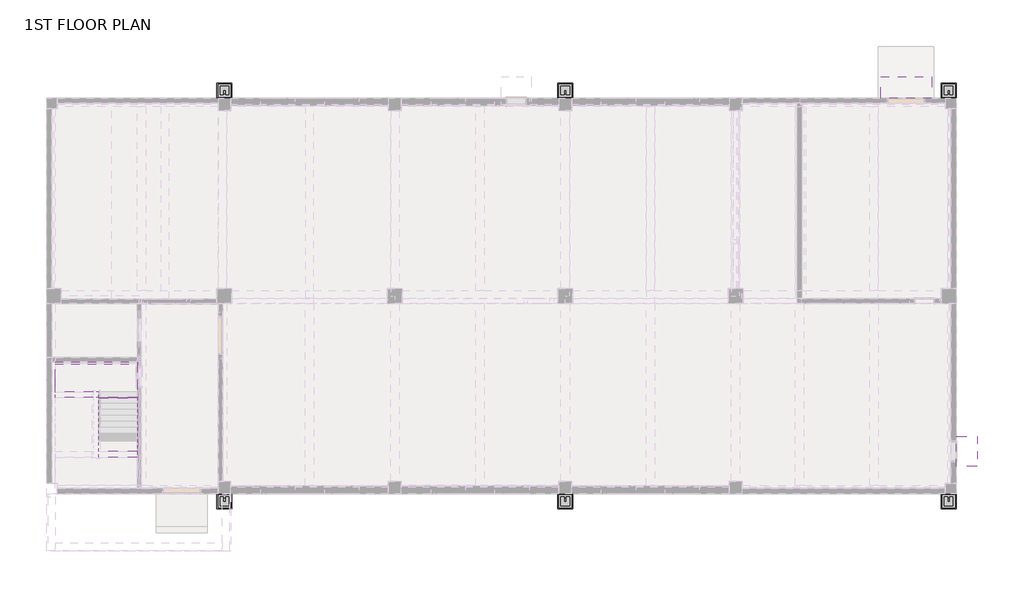
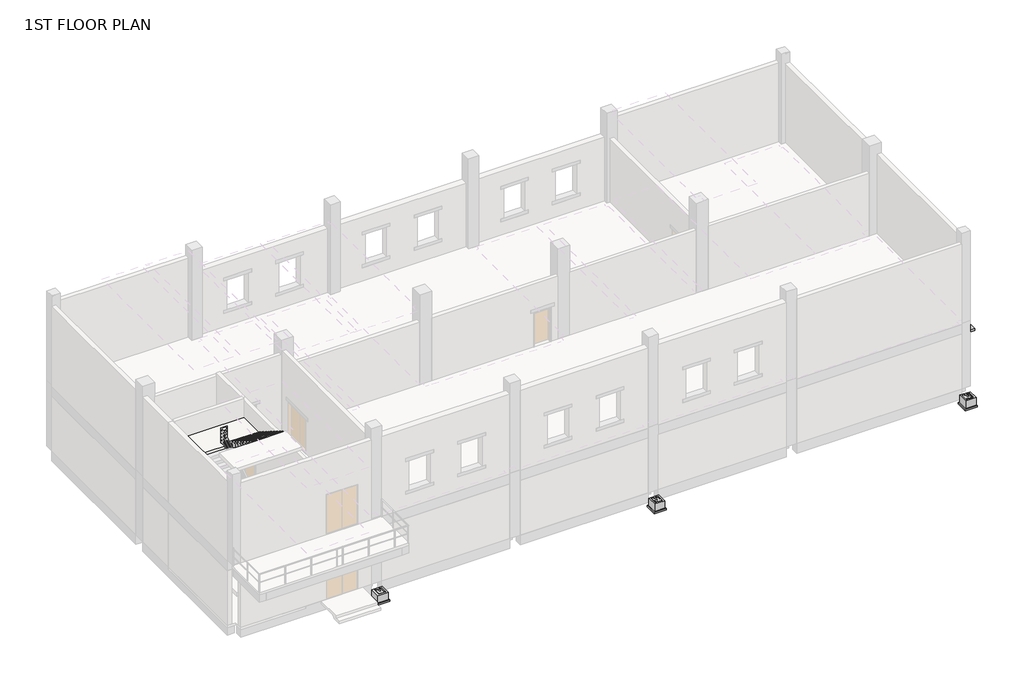
# One storey, part 9 of 9: 8 proxies, 2 slabs, 2 stair flights.
"""IFC4 building model written with IfcOpenShell, lengths in millimetres."""

import ifcopenshell
import ifcopenshell.guid

model = None  # the IFC model being written
_history = None  # IfcOwnerHistory: only IFC2X3 demands one
_inside = {}  # id of a spatial element -> (the spatial element, [elements in it])
_under = {}  # id of a project, library or spatial element -> (it, [spatial elements below it])
_declared = {}  # id of a project -> (the project, [libraries it declares])
_typed = {}  # id of a type object -> (the type object, [elements of that type])
_made_of = {}  # id of a material, layer set ... -> (it, [elements and type objects made of it])


def new_model(schema):
    """Start an empty IFC model of exactly this schema.

    Asked for "IFC4X3", IfcOpenShell would pick the latest addendum, in which some entities
    have other attributes; the version numbers below select the first issue.
    IFC2X3 requires an IfcOwnerHistory on every rooted entity: one is made here for all.
    """
    global model, _history
    if schema == "IFC4X3":
        model = ifcopenshell.file(schema_version=(4, 3, 0, 0))
    else:
        model = ifcopenshell.file(schema=schema)
    _inside.clear()
    _under.clear()
    _declared.clear()
    _typed.clear()
    _made_of.clear()
    _history = None
    if model.schema == "IFC2X3":
        org = make("IfcOrganization", Name="unknown")
        user = make(
            "IfcPersonAndOrganization",
            ThePerson=make("IfcPerson", FamilyName="unknown"),
            TheOrganization=org,
        )
        app = make(
            "IfcApplication",
            ApplicationDeveloper=org,
            Version="unknown",
            ApplicationFullName="unknown",
            ApplicationIdentifier="unknown",
        )
        _history = make(
            "IfcOwnerHistory",
            OwningUser=user,
            OwningApplication=app,
            ChangeAction="ADDED",
            CreationDate=0,
        )
    return model


def make(cls, **values):
    """One entity of the class cls with the attributes given. An attribute that is None is left unset."""
    return model.create_entity(
        cls, **{name: value for name, value in values.items() if value is not None}
    )


def rooted(cls, **values):
    """An entity with a GlobalId (a new one), such as an element, a storey or a relation."""
    return make(cls, GlobalId=ifcopenshell.guid.new(), OwnerHistory=_history, **values)


def si_unit(unit_type, name, prefix=None):
    """IfcSIUnit, for example si_unit("LENGTHUNIT", "METRE", prefix="MILLI")."""
    return make("IfcSIUnit", UnitType=unit_type, Prefix=prefix, Name=name)


def assignment(units):
    """IfcUnitAssignment: the units of a project."""
    return None if units is None else make("IfcUnitAssignment", Units=units)


def point(xyz):
    """IfcCartesianPoint."""
    return None if xyz is None else make("IfcCartesianPoint", Coordinates=xyz)


def direction(xyz):
    """IfcDirection."""
    return None if xyz is None else make("IfcDirection", DirectionRatios=xyz)


def frame(location, z_axis=None, x_axis=None):
    """IfcAxis2Placement3D, a coordinate frame: its origin and axes. An axis left out is left unset."""
    return make(
        "IfcAxis2Placement3D",
        Location=point(location),
        Axis=direction(z_axis),
        RefDirection=direction(x_axis),
    )


def origin():
    """The frame at (0, 0, 0) with its axes left unset."""
    return frame((0.0, 0.0, 0.0))


def origin_with_axes():
    """The frame at (0, 0, 0) with the z axis (0, 0, 1) and the x axis (1, 0, 0) written out."""
    return frame((0.0, 0.0, 0.0), z_axis=(0.0, 0.0, 1.0), x_axis=(1.0, 0.0, 0.0))


def place(relative_to, where):
    """IfcLocalPlacement: puts the frame where relative to a parent placement (None: the world)."""
    return make(
        "IfcLocalPlacement", PlacementRelTo=relative_to, RelativePlacement=where
    )


def context(
    kind, dimensions, precision=None, world=None, true_north=None, identifier=None
):
    """IfcGeometricRepresentationContext, for example the 3D "Model" context."""
    return make(
        "IfcGeometricRepresentationContext",
        ContextIdentifier=identifier,
        ContextType=kind,
        CoordinateSpaceDimension=dimensions,
        Precision=precision,
        WorldCoordinateSystem=world,
        TrueNorth=true_north,
    )


def project(units=None, contexts=None):
    """IfcProject with its units and contexts."""
    return rooted(
        "IfcProject",
        Name="project",
        RepresentationContexts=contexts,
        UnitsInContext=assignment(units),
    )


def spatial(cls, under=None, at=None, **own):
    """A site, building, storey or space (cls), placed at a placement, below another one or the project."""
    s = rooted(cls, ObjectPlacement=at, **own)
    if under is not None:
        _under.setdefault(under.id(), (under, []))[1].append(s)
    return s


def polyline(points):
    """IfcPolyline through the points."""
    return make("IfcPolyline", Points=[point(p) for p in points])


def outline(outer, holes=None, kind="AREA"):
    """IfcArbitraryClosedProfileDef: a profile drawn as a closed curve; with holes, ...WithVoids."""
    if holes is None:
        return make("IfcArbitraryClosedProfileDef", ProfileType=kind, OuterCurve=outer)
    return make(
        "IfcArbitraryProfileDefWithVoids",
        ProfileType=kind,
        OuterCurve=outer,
        InnerCurves=holes,
    )


def extrude(swept, where, along, depth):
    """IfcExtrudedAreaSolid: the profile swept, set in the frame where, extruded along a direction by depth."""
    return make(
        "IfcExtrudedAreaSolid",
        SweptArea=swept,
        Position=where,
        ExtrudedDirection=direction(along),
        Depth=depth,
    )


def faces_of(points, faces, orient=None, outer=None):
    """IfcFace entities. A face is a list of loops; a loop is a list of indices into points, from 0.

    orient and outer hold one flag for each loop. By default every Orientation is true, the
    first loop of a face is its IfcFaceOuterBound and the others are IfcFaceBound.
    """
    made = []
    for i, loops in enumerate(faces):
        bounds = []
        for j, loop in enumerate(loops):
            is_outer = j == 0 if outer is None else outer[i][j]
            bounds.append(
                make(
                    "IfcFaceOuterBound" if is_outer else "IfcFaceBound",
                    Bound=make("IfcPolyLoop", Polygon=[points[k] for k in loop]),
                    Orientation=True if orient is None else orient[i][j],
                )
            )
        made.append(make("IfcFace", Bounds=bounds))
    return made


def faceted_brep(points, faces, orient=None, outer=None, voids=None):
    """IfcFacetedBrep: a solid bounded by flat faces; with voids (closed shells), ...WithVoids."""
    shared = [point(p) for p in points]
    hull = make("IfcClosedShell", CfsFaces=faces_of(shared, faces, orient, outer))
    if voids is None:
        return make("IfcFacetedBrep", Outer=hull)
    return make(
        "IfcFacetedBrepWithVoids",
        Outer=hull,
        Voids=[
            make(cls, CfsFaces=faces_of(shared, fs, o, b)) for cls, fs, o, b in voids
        ],
    )


def shape(context_of_items, identifier, shape_type, items):
    """IfcShapeRepresentation: the items that make up one representation, for example the "Body"."""
    return make(
        "IfcShapeRepresentation",
        ContextOfItems=context_of_items,
        RepresentationIdentifier=identifier,
        RepresentationType=shape_type,
        Items=items,
    )


def source(mapping_origin, context_of_items, identifier, shape_type, items):
    """IfcRepresentationMap: a shape defined once, which mapped items show again and again."""
    return make(
        "IfcRepresentationMap",
        MappingOrigin=mapping_origin,
        MappedRepresentation=shape(context_of_items, identifier, shape_type, items),
    )


def transform(
    local_origin,
    x_axis=None,
    y_axis=None,
    z_axis=None,
    scale=None,
    scale2=None,
    scale3=None,
    uniform=True,
):
    """IfcCartesianTransformationOperator3D, or its non-uniform kind. x_axis, y_axis, z_axis: its Axis1, 2, 3."""
    if uniform:
        return make(
            "IfcCartesianTransformationOperator3D",
            Axis1=direction(x_axis),
            Axis2=direction(y_axis),
            LocalOrigin=point(local_origin),
            Scale=scale,
            Axis3=direction(z_axis),
        )
    return make(
        "IfcCartesianTransformationOperator3DnonUniform",
        Axis1=direction(x_axis),
        Axis2=direction(y_axis),
        LocalOrigin=point(local_origin),
        Scale=scale,
        Axis3=direction(z_axis),
        Scale2=scale2,
        Scale3=scale3,
    )


def mapped(mapping_source, mapping_target):
    """IfcMappedItem: shows the shape of a source again, moved by a transform."""
    return make(
        "IfcMappedItem", MappingSource=mapping_source, MappingTarget=mapping_target
    )


def made_of(thing, what):
    """Note that an element or type object is made of a material, layer set ...; save() writes the relation."""
    if what is not None:
        _made_of.setdefault(what.id(), (what, []))[1].append(thing)
    return thing


def element(
    cls,
    number,
    at=None,
    inside=None,
    cuts=None,
    type_object=None,
    material=None,
    context=None,
    identifier="Body",
    shape_type=None,
    held_by="IfcProductDefinitionShape",
    body=None,
    shapes=None,
    **own,
):
    """One element of the class cls, such as IfcWall. Its Tag is "e" and its number.

    at: its placement. inside: the storey or other place that contains it. cuts: it is an
    opening in that element (IfcRelVoidsElement). A single representation is given by context,
    identifier, shape_type and body (its items); several are given by shapes. held_by: the class
    of the entity that holds the representations. save() writes the other relations.
    """
    e = rooted(cls, Tag="e%d" % number, ObjectPlacement=at, **own)
    if body is not None:
        shapes = [shape(context, identifier, shape_type, body)]
    if shapes is not None:
        e.Representation = make(held_by, Representations=shapes)
    if inside is not None:
        _inside.setdefault(inside.id(), (inside, []))[1].append(e)
    if cuts is not None:
        rooted(
            "IfcRelVoidsElement", RelatingBuildingElement=cuts, RelatedOpeningElement=e
        )
    if type_object is not None:
        _typed.setdefault(type_object.id(), (type_object, []))[1].append(e)
    return made_of(e, material)


def aggregate(whole, parts):
    """IfcRelAggregates: a whole, such as a stair, and the parts it consists of."""
    return rooted("IfcRelAggregates", RelatingObject=whole, RelatedObjects=parts)


def save(model, path):
    """Write the relations noted so far, then the file.

    IfcRelAggregates (storeys below a building ...), IfcRelContainedInSpatialStructure (elements
    in a storey), IfcRelDefinesByType, IfcRelAssociatesMaterial and IfcRelDeclares: one each for
    every whole, place, type object, material and project.
    """
    for whole, parts in _under.values():
        aggregate(whole, parts)
    for where, things in _inside.values():
        rooted(
            "IfcRelContainedInSpatialStructure",
            RelatedElements=things,
            RelatingStructure=where,
        )
    for kind, things in _typed.values():
        rooted("IfcRelDefinesByType", RelatedObjects=things, RelatingType=kind)
    for what, things in _made_of.values():
        rooted("IfcRelAssociatesMaterial", RelatedObjects=things, RelatingMaterial=what)
    for by, libraries in _declared.values():
        rooted("IfcRelDeclares", RelatingContext=by, RelatedDefinitions=libraries)
    model.write(path)


def generic_models_4b8b6a59(model_context):
    return source(origin(), model_context, "Body", "SolidModel", [
        extrude(outline(polyline([(-55.0, 140.0), (-55.0, 132.0), (-132.0, 132.0), (-132.0, -132.0), (132.0, -132.0), (132.0, 132.0), (55.0, 132.0), (55.0, 140.0), (140.0, 140.0), (140.0, -140.0), (-140.0, -140.0), (-140.0, 140.0), (-55.0, 140.0)])), frame((0.0, 0.0, -10.0), z_axis=(0.0, 0.0, 1.0), x_axis=(1.0, 0.0, 0.0)), (0.0, 0.0, 1.0), 10.0),
        extrude(outline(polyline([(-55.0, 200.0), (-55.0, -20.0), (55.0, -20.0), (55.0, 200.0), (200.0, 200.0), (200.0, -200.0), (-200.0, -200.0), (-200.0, 200.0), (-55.0, 200.0)])), origin_with_axes(), (0.0, 0.0, 1.0), 8.0),
        faceted_brep([(150.0, -150.0, -300.0), (150.0, 150.0, -300.0), (-150.0, 150.0, -300.0), (-150.0, -150.0, -300.0), (300.0, 300.0, -450.0), (300.0, -300.0, -450.0), (-300.0, -300.0, -450.0), (-300.0, 300.0, -450.0), (-300.0, 300.0, 0.0), (300.0, 300.0, 0.0), (-300.0, -300.0, 0.0), (300.0, -300.0, 0.0), (150.0, 150.0, 0.0), (150.0, -150.0, 0.0), (-150.0, -150.0, 0.0), (-150.0, 150.0, 0.0)], [[[0, 1, 2, 3]], [[4, 5, 6, 7]], [[4, 7, 8, 9]], [[8, 7, 6, 10]], [[10, 6, 5, 11]], [[11, 5, 4, 9]], [[9, 8, 10, 11], [12, 13, 14, 15]], [[13, 12, 1, 0]], [[14, 13, 0, 3]], [[15, 14, 3, 2]], [[12, 15, 2, 1]]]),
        extrude(outline(polyline([(350.0, 350.0), (350.0, -350.0), (-350.0, -350.0), (-350.0, 350.0), (350.0, 350.0)])), frame((0.0, 0.0, -550.0), z_axis=(0.0, 0.0, 1.0), x_axis=(1.0, 0.0, 0.0)), (0.0, 0.0, 1.0), 100.0),
    ])


def generic_models_1eaa761a(model_context):
    return source(origin(), model_context, "Body", "SolidModel", [
        extrude(outline(polyline([(-55.0, -140.0), (-140.0, -140.0), (-140.0, 140.0), (140.0, 140.0), (140.0, -140.0), (55.0, -140.0), (55.0, -132.0), (132.0, -132.0), (132.0, 132.0), (-132.0, 132.0), (-132.0, -132.0), (-55.0, -132.0), (-55.0, -140.0)])), frame((0.0, 0.0, -10.0), z_axis=(0.0, 0.0, 1.0), x_axis=(1.0, 0.0, 0.0)), (0.0, 0.0, 1.0), 10.0),
        extrude(outline(polyline([(-55.0, -200.0), (-200.0, -200.0), (-200.0, 200.0), (200.0, 200.0), (200.0, -200.0), (55.0, -200.0), (55.0, 20.0), (-55.0, 20.0), (-55.0, -200.0)])), origin_with_axes(), (0.0, 0.0, 1.0), 8.0),
        faceted_brep([(150.0, 150.0, -300.0), (-150.0, 150.0, -300.0), (-150.0, -150.0, -300.0), (150.0, -150.0, -300.0), (300.0, -300.0, -450.0), (-300.0, -300.0, -450.0), (-300.0, 300.0, -450.0), (300.0, 300.0, -450.0), (300.0, -300.0, 0.0), (-300.0, -300.0, 0.0), (-300.0, 300.0, 0.0), (300.0, 300.0, 0.0), (150.0, -150.0, 0.0), (-150.0, -150.0, 0.0), (-150.0, 150.0, 0.0), (150.0, 150.0, 0.0)], [[[0, 1, 2, 3]], [[4, 5, 6, 7]], [[4, 8, 9, 5]], [[9, 10, 6, 5]], [[10, 11, 7, 6]], [[11, 8, 4, 7]], [[8, 11, 10, 9], [12, 13, 14, 15]], [[15, 0, 3, 12]], [[14, 1, 0, 15]], [[13, 2, 1, 14]], [[12, 3, 2, 13]]]),
        extrude(outline(polyline([(350.0, -350.0), (-350.0, -350.0), (-350.0, 350.0), (350.0, 350.0), (350.0, -350.0)])), frame((0.0, 0.0, -550.0), z_axis=(0.0, 0.0, 1.0), x_axis=(1.0, 0.0, 0.0)), (0.0, 0.0, 1.0), 100.0),
    ])


def canopy_no_lintel2_canopy_no_lintel_90d8ac49(model_context):
    return source(origin(), model_context, "Body", "SweptSolid", [
        extrude(outline(polyline([(-30.0, 1000.0), (0.0, 0.0), (-150.0, 0.0), (-150.0, 1000.0), (-30.0, 1000.0)])), frame((0.0, 0.0, 0.0), z_axis=(1.0, 0.0, 0.0), x_axis=(0.0, 1.0, 0.0)), (0.0, 0.0, 1.0), 1400.0),
    ])


def canopy_no_lintel2_canopy_no_lintel_c6626c79(model_context):
    return source(origin(), model_context, "Body", "SweptSolid", [
        extrude(outline(polyline([(-30.0, 1000.0), (0.0, 0.0), (-150.0, 0.0), (-150.0, 1000.0), (-30.0, 1000.0)])), frame((0.0, 0.0, 0.0), z_axis=(1.0, 0.0, 0.0), x_axis=(0.0, 1.0, 0.0)), (0.0, 0.0, 1.0), 2400.0),
    ])


model = new_model("IFC4")

# Units and contexts
model_context = context("Model", 3, world=origin())
ifc_project = project(units=[si_unit("LENGTHUNIT", "METRE", prefix="MILLI")], contexts=[model_context])

# Site, building, storey
site = spatial("IfcSite", under=ifc_project)
building = spatial("IfcBuilding", under=site)
storey = spatial("IfcBuildingStorey", under=building, Name="1ST FLOOR PLAN", Elevation=600.005241)

# Proxies
placement = place(None, origin())
generic_models_shape = generic_models_4b8b6a59(model_context)
element("IfcBuildingElementProxy", 1, Name="Catchpit : Rainwater Catchpit", ObjectType="Catchpit : Rainwater Catchpit", at=placement, inside=storey, context=model_context, shape_type="MappedRepresentation", body=[
    mapped(generic_models_shape, transform((8000.0, 20349.4942467, 300.005241), x_axis=(1.0, 0.0, 0.0), y_axis=(0.0, 1.0, 0.0), z_axis=(0.0, 0.0, 1.0))),
])
element("IfcBuildingElementProxy", 2, Name="Catchpit : Rainwater Catchpit", ObjectType="Catchpit : Rainwater Catchpit", at=placement, inside=storey, context=model_context, shape_type="MappedRepresentation", body=[
    mapped(generic_models_shape, transform((24000.0, 20349.4942467, 300.005241), x_axis=(1.0, 0.0, 0.0), y_axis=(0.0, 1.0, 0.0), z_axis=(0.0, 0.0, 1.0))),
])
element("IfcBuildingElementProxy", 3, Name="Catchpit : Rainwater Catchpit", ObjectType="Catchpit : Rainwater Catchpit", at=placement, inside=storey, context=model_context, shape_type="MappedRepresentation", body=[
    mapped(generic_models_shape, transform((42000.0, 20349.4942467, 300.005241), x_axis=(1.0, 0.0, 0.0), y_axis=(0.0, 1.0, 0.0), z_axis=(0.0, 0.0, 1.0))),
])
generic_models_2_shape = generic_models_1eaa761a(model_context)
element("IfcBuildingElementProxy", 4, Name="Catchpit : Rainwater Catchpit", ObjectType="Catchpit : Rainwater Catchpit", at=placement, inside=storey, context=model_context, shape_type="MappedRepresentation", body=[
    mapped(generic_models_2_shape, transform((8000.0, 39649.5474711, 300.005241), x_axis=(1.0, 0.0, 0.0), y_axis=(0.0, 1.0, 0.0), z_axis=(0.0, 0.0, 1.0))),
])
element("IfcBuildingElementProxy", 5, Name="Catchpit : Rainwater Catchpit", ObjectType="Catchpit : Rainwater Catchpit", at=placement, inside=storey, context=model_context, shape_type="MappedRepresentation", body=[
    mapped(generic_models_2_shape, transform((24000.0, 39649.5474711, 300.005241), x_axis=(1.0, 0.0, 0.0), y_axis=(0.0, 1.0, 0.0), z_axis=(0.0, 0.0, 1.0))),
])
element("IfcBuildingElementProxy", 6, Name="Catchpit : Rainwater Catchpit", ObjectType="Catchpit : Rainwater Catchpit", at=placement, inside=storey, context=model_context, shape_type="MappedRepresentation", body=[
    mapped(generic_models_2_shape, transform((42000.0, 39649.5474711, 300.005241), x_axis=(1.0, 0.0, 0.0), y_axis=(0.0, 1.0, 0.0), z_axis=(0.0, 0.0, 1.0))),
])
canopy_no_lintel2_canopy_no_lintel_shape = canopy_no_lintel2_canopy_no_lintel_90d8ac49(model_context)
element("IfcBuildingElementProxy", 7, Name="Canopy_no_ Lintel2 : Canopy No Lintel", ObjectType="Canopy_no_ Lintel2 : Canopy No Lintel", at=placement, inside=storey, context=model_context, shape_type="MappedRepresentation", body=[
    mapped(canopy_no_lintel2_canopy_no_lintel_shape, transform((42351.0, 21999.5208589, 3000.005241), x_axis=(0.0, 1.0, 0.0), y_axis=(0.0, 0.0, 1.0), z_axis=(1.0, 0.0, 0.0))),
])
canopy_no_lintel2_canopy_no_lintel_2_shape = canopy_no_lintel2_canopy_no_lintel_c6626c79(model_context)
element("IfcBuildingElementProxy", 8, Name="Canopy_no_ Lintel2 : Canopy No Lintel", ObjectType="Canopy_no_ Lintel2 : Canopy No Lintel", at=placement, inside=storey, context=model_context, shape_type="MappedRepresentation", body=[
    mapped(canopy_no_lintel2_canopy_no_lintel_2_shape, transform((41200.0, 39300.5208589, 3400.005241), x_axis=(-1.0, 0.0, 0.0), y_axis=(0.0, 0.0, 1.0), z_axis=(0.0, 1.0, 0.0))),
])

# Slabs
element("IfcSlab", 9, ObjectType="프리캐스트 콘크리트 - 200mm 두께", at=placement, inside=storey, context=model_context, shape_type="SolidModel", body=[
    faceted_brep([(50.0, 25499.5208589, 4599.211491), (1850.0, 25499.5208589, 4599.211491), (2100.0, 25499.5208589, 4599.211491), (2100.0, 25219.5208589, 4599.211491), (3900.0, 25219.5208589, 4599.211491), (3900.0, 26799.5208589, 4599.211491), (50.0, 26799.5208589, 4599.211491), (50.0, 25736.7852447, 4599.211491), (3900.0, 25219.5208589, 4399.211491), (3900.0, 26799.5208589, 4399.211491), (50.0, 26799.5208589, 4399.211491), (50.0, 25499.5208589, 4257.9826899), (50.0, 25499.5208589, 4432.5448243), (50.0, 25736.7852447, 4399.211491), (1850.0, 25736.7852447, 4399.211491), (2100.0, 25219.5208589, 4399.211491), (2100.0, 25499.5208589, 4399.211491), (1850.0, 25499.5208589, 4399.211491), (1850.0, 25499.5208589, 4257.9826899)], [[[0, 1, 2, 3, 4, 5, 6, 7]], [[5, 4, 8, 9]], [[6, 5, 9, 10]], [[11, 12, 0, 7, 6, 10, 13]], [[14, 13, 10, 9, 8, 15, 16, 17]], [[1, 0, 12, 11, 18, 17]], [[2, 1, 17, 16]], [[13, 14, 18, 11]], [[14, 17, 18]], [[3, 2, 16, 15]], [[4, 3, 15, 8]]]),
    extrude(outline(polyline([(50.0, 25499.5208589), (50.0, 26799.5208589), (3900.0, 26799.5208589), (3900.0, 25219.5208589), (2100.0, 25219.5208589), (2100.0, 25499.5208589), (1850.0, 25499.5208589), (50.0, 25499.5208589)])), frame((0.0, 0.0, 4599.211491), z_axis=(0.0, 0.0, 1.0), x_axis=(1.0, 0.0, 0.0)), (0.0, 0.0, 1.0), 0.79375),
])
element("IfcSlab", 10, ObjectType="프리캐스트 콘크리트 - 200mm 두께", at=placement, inside=storey, context=model_context, shape_type="SolidModel", body=[
    faceted_brep([(50.0, 25219.5208589, 8380.461491), (1850.0, 25219.5208589, 8380.461491), (2100.0, 25219.5208589, 8380.461491), (3900.0, 25219.5208589, 8380.461491), (3900.0, 25258.6099233, 8380.461491), (3900.0, 26899.5208589, 8380.461491), (50.0, 26899.5208589, 8380.461491), (50.0, 25460.4317945, 8380.461491), (50.0, 25219.5208589, 8208.586491), (50.0, 25219.5208589, 8032.5808943), (1850.0, 25219.5208589, 8032.5808943), (1850.0, 25219.5208589, 8180.461491), (2100.0, 25219.5208589, 8180.461491), (2100.0, 25219.5208589, 8204.4558943), (3900.0, 25219.5208589, 8204.4558943), (3900.0, 25258.6099233, 8180.461491), (3900.0, 26899.5208589, 8180.461491), (50.0, 26899.5208589, 8180.461491), (50.0, 25460.4317945, 8180.461491), (2100.0, 25258.6099233, 8180.461491), (1850.0, 25460.4317945, 8180.461491)], [[[0, 1, 2, 3, 4, 5, 6, 7]], [[1, 0, 8, 9, 10, 11]], [[2, 1, 11, 12, 13]], [[3, 2, 13, 14]], [[3, 14, 15, 16, 5, 4]], [[6, 5, 16, 17]], [[9, 8, 0, 7, 6, 17, 18]], [[19, 12, 11, 20, 18, 17, 16, 15]], [[12, 19, 13]], [[18, 20, 10, 9]], [[20, 11, 10]], [[19, 15, 14, 13]]]),
    extrude(outline(polyline([(50.0, 25219.5208589), (50.0, 26899.5208589), (3900.0, 26899.5208589), (3900.0, 25219.5208589), (2100.0, 25219.5208589), (1850.0, 25219.5208589), (50.0, 25219.5208589)])), frame((0.0, 0.0, 8380.461491), z_axis=(0.0, 0.0, 1.0), x_axis=(1.0, 0.0, 0.0)), (0.0, 0.0, 1.0), 0.79375),
])

# Stair flights
element("IfcStairFlight", 11, ObjectType="1mm 디딤판", at=placement, inside=storey, context=model_context, shape_type="SolidModel", body=[
    faceted_brep([(3900.0, 24939.5208589, 4771.086491), (3900.0, 25219.5208589, 4771.086491), (2100.0, 25219.5208589, 4771.086491), (2100.0, 24939.5208589, 4771.086491), (3900.0, 24939.5208589, 4600.005241), (3900.0, 25219.5208589, 4600.005241), (2100.0, 25219.5208589, 4600.005241), (2100.0, 24939.5208589, 4600.005241), (3900.0, 24659.5208589, 4942.961491), (3900.0, 24939.5208589, 4942.961491), (2100.0, 24939.5208589, 4942.961491), (2100.0, 24659.5208589, 4942.961491), (3900.0, 24659.5208589, 4766.9558943), (3900.0, 24931.4986506, 4600.005241), (2100.0, 24931.4986506, 4600.005241), (2100.0, 24659.5208589, 4766.9558943), (3900.0, 24379.5208589, 5114.836491), (3900.0, 24659.5208589, 5114.836491), (2100.0, 24659.5208589, 5114.836491), (2100.0, 24379.5208589, 5114.836491), (3900.0, 24379.5208589, 4938.8308943), (2100.0, 24379.5208589, 4938.8308943), (3900.0, 24099.5208589, 5286.711491), (3900.0, 24379.5208589, 5286.711491), (2100.0, 24379.5208589, 5286.711491), (2100.0, 24099.5208589, 5286.711491), (3900.0, 24099.5208589, 5110.7058943), (2100.0, 24099.5208589, 5110.7058943), (3900.0, 23819.5208589, 5458.586491), (3900.0, 24099.5208589, 5458.586491), (2100.0, 24099.5208589, 5458.586491), (2100.0, 23819.5208589, 5458.586491), (3900.0, 23819.5208589, 5282.5808943), (2100.0, 23819.5208589, 5282.5808943), (3900.0, 23539.5208589, 5630.461491), (3900.0, 23819.5208589, 5630.461491), (2100.0, 23819.5208589, 5630.461491), (2100.0, 23539.5208589, 5630.461491), (3900.0, 23539.5208589, 5454.4558943), (2100.0, 23539.5208589, 5454.4558943), (3900.0, 23259.5208589, 5802.336491), (3900.0, 23539.5208589, 5802.336491), (2100.0, 23539.5208589, 5802.336491), (2100.0, 23259.5208589, 5802.336491), (3900.0, 23259.5208589, 5626.3308943), (2100.0, 23259.5208589, 5626.3308943), (3900.0, 22979.5208589, 5974.211491), (3900.0, 23259.5208589, 5974.211491), (2100.0, 23259.5208589, 5974.211491), (2100.0, 22979.5208589, 5974.211491), (3900.0, 22979.5208589, 5798.2058943), (2100.0, 22979.5208589, 5798.2058943), (3900.0, 22699.5208589, 6146.086491), (3900.0, 22979.5208589, 6146.086491), (2100.0, 22979.5208589, 6146.086491), (2100.0, 22699.5208589, 6146.086491), (3900.0, 22699.5208589, 5970.0808943), (2100.0, 22699.5208589, 5970.0808943), (3900.0, 22419.5208589, 6317.961491), (3900.0, 22699.5208589, 6317.961491), (2100.0, 22699.5208589, 6317.961491), (2100.0, 22419.5208589, 6317.961491), (3900.0, 22419.5208589, 6141.9558943), (2100.0, 22419.5208589, 6141.9558943), (2100.0, 22419.5208589, 6289.836491)], [[[0, 1, 2, 3]], [[1, 0, 4, 5]], [[2, 1, 5, 6]], [[3, 2, 6, 7]], [[8, 9, 10, 11]], [[4, 0, 9, 8, 12, 13]], [[0, 3, 10, 9]], [[3, 7, 14, 15, 11, 10]], [[16, 17, 18, 19]], [[17, 16, 20, 12, 8]], [[8, 11, 18, 17]], [[19, 18, 11, 15, 21]], [[22, 23, 24, 25]], [[23, 22, 26, 20, 16]], [[16, 19, 24, 23]], [[25, 24, 19, 21, 27]], [[28, 29, 30, 31]], [[29, 28, 32, 26, 22]], [[22, 25, 30, 29]], [[31, 30, 25, 27, 33]], [[34, 35, 36, 37]], [[35, 34, 38, 32, 28]], [[28, 31, 36, 35]], [[37, 36, 31, 33, 39]], [[40, 41, 42, 43]], [[41, 40, 44, 38, 34]], [[34, 37, 42, 41]], [[43, 42, 37, 39, 45]], [[46, 47, 48, 49]], [[47, 46, 50, 44, 40]], [[40, 43, 48, 47]], [[49, 48, 43, 45, 51]], [[52, 53, 54, 55]], [[53, 52, 56, 50, 46]], [[46, 49, 54, 53]], [[55, 54, 49, 51, 57]], [[58, 59, 60, 61]], [[59, 58, 62, 56, 52]], [[52, 55, 60, 59]], [[61, 60, 55, 57, 63, 64]], [[58, 61, 64, 63, 62]], [[5, 4, 13, 14, 7, 6]], [[14, 13, 12, 20, 26, 32, 38, 44, 50, 56, 62, 63, 57, 51, 45, 39, 33, 27, 21, 15]]]),
    extrude(outline(polyline([(3900.0, 24939.5208589), (2100.0, 24939.5208589), (2100.0, 25219.5208589), (3900.0, 25219.5208589), (3900.0, 24939.5208589)])), frame((0.0, 0.0, 4771.086491), z_axis=(0.0, 0.0, 1.0), x_axis=(1.0, 0.0, 0.0)), (0.0, 0.0, 1.0), 0.79375),
    extrude(outline(polyline([(3900.0, 24659.5208589), (2100.0, 24659.5208589), (2100.0, 24939.5208589), (3900.0, 24939.5208589), (3900.0, 24659.5208589)])), frame((0.0, 0.0, 4942.961491), z_axis=(0.0, 0.0, 1.0), x_axis=(1.0, 0.0, 0.0)), (0.0, 0.0, 1.0), 0.79375),
    extrude(outline(polyline([(3900.0, 24379.5208589), (2100.0, 24379.5208589), (2100.0, 24659.5208589), (3900.0, 24659.5208589), (3900.0, 24379.5208589)])), frame((0.0, 0.0, 5114.836491), z_axis=(0.0, 0.0, 1.0), x_axis=(1.0, 0.0, 0.0)), (0.0, 0.0, 1.0), 0.79375),
    extrude(outline(polyline([(3900.0, 24099.5208589), (2100.0, 24099.5208589), (2100.0, 24379.5208589), (3900.0, 24379.5208589), (3900.0, 24099.5208589)])), frame((0.0, 0.0, 5286.711491), z_axis=(0.0, 0.0, 1.0), x_axis=(1.0, 0.0, 0.0)), (0.0, 0.0, 1.0), 0.79375),
    extrude(outline(polyline([(3900.0, 23819.5208589), (2100.0, 23819.5208589), (2100.0, 24099.5208589), (3900.0, 24099.5208589), (3900.0, 23819.5208589)])), frame((0.0, 0.0, 5458.586491), z_axis=(0.0, 0.0, 1.0), x_axis=(1.0, 0.0, 0.0)), (0.0, 0.0, 1.0), 0.79375),
    extrude(outline(polyline([(3900.0, 23539.5208589), (2100.0, 23539.5208589), (2100.0, 23819.5208589), (3900.0, 23819.5208589), (3900.0, 23539.5208589)])), frame((0.0, 0.0, 5630.461491), z_axis=(0.0, 0.0, 1.0), x_axis=(1.0, 0.0, 0.0)), (0.0, 0.0, 1.0), 0.79375),
    extrude(outline(polyline([(3900.0, 23259.5208589), (2100.0, 23259.5208589), (2100.0, 23539.5208589), (3900.0, 23539.5208589), (3900.0, 23259.5208589)])), frame((0.0, 0.0, 5802.336491), z_axis=(0.0, 0.0, 1.0), x_axis=(1.0, 0.0, 0.0)), (0.0, 0.0, 1.0), 0.79375),
    extrude(outline(polyline([(3900.0, 22979.5208589), (2100.0, 22979.5208589), (2100.0, 23259.5208589), (3900.0, 23259.5208589), (3900.0, 22979.5208589)])), frame((0.0, 0.0, 5974.211491), z_axis=(0.0, 0.0, 1.0), x_axis=(1.0, 0.0, 0.0)), (0.0, 0.0, 1.0), 0.79375),
    extrude(outline(polyline([(3900.0, 22699.5208589), (2100.0, 22699.5208589), (2100.0, 22979.5208589), (3900.0, 22979.5208589), (3900.0, 22699.5208589)])), frame((0.0, 0.0, 6146.086491), z_axis=(0.0, 0.0, 1.0), x_axis=(1.0, 0.0, 0.0)), (0.0, 0.0, 1.0), 0.79375),
    extrude(outline(polyline([(3900.0, 22419.5208589), (2100.0, 22419.5208589), (2100.0, 22699.5208589), (3900.0, 22699.5208589), (3900.0, 22419.5208589)])), frame((0.0, 0.0, 6317.961491), z_axis=(0.0, 0.0, 1.0), x_axis=(1.0, 0.0, 0.0)), (0.0, 0.0, 1.0), 0.79375),
])
element("IfcStairFlight", 12, ObjectType="1mm 디딤판", at=placement, inside=storey, context=model_context, shape_type="SolidModel", body=[
    faceted_brep([(3900.0, 24939.5208589, 8552.336491), (3900.0, 25219.5208589, 8552.336491), (2100.0, 25219.5208589, 8552.336491), (2100.0, 24939.5208589, 8552.336491), (3900.0, 24939.5208589, 8376.3308943), (3900.0, 25219.5208589, 8204.4558943), (3900.0, 25219.5208589, 8380.461491), (2100.0, 25219.5208589, 8204.4558943), (2100.0, 24939.5208589, 8376.3308943), (3900.0, 24659.5208589, 8724.211491), (3900.0, 24939.5208589, 8724.211491), (2100.0, 24939.5208589, 8724.211491), (2100.0, 24659.5208589, 8724.211491), (3900.0, 24659.5208589, 8548.2058943), (2100.0, 24659.5208589, 8548.2058943), (3900.0, 24379.5208589, 8896.086491), (3900.0, 24659.5208589, 8896.086491), (2100.0, 24659.5208589, 8896.086491), (2100.0, 24379.5208589, 8896.086491), (3900.0, 24379.5208589, 8720.0808943), (2100.0, 24379.5208589, 8720.0808943), (3900.0, 24099.5208589, 9067.961491), (3900.0, 24379.5208589, 9067.961491), (2100.0, 24379.5208589, 9067.961491), (2100.0, 24099.5208589, 9067.961491), (3900.0, 24099.5208589, 8891.9558943), (2100.0, 24099.5208589, 8891.9558943), (3900.0, 23819.5208589, 9239.836491), (3900.0, 24099.5208589, 9239.836491), (2100.0, 24099.5208589, 9239.836491), (2100.0, 23819.5208589, 9239.836491), (3900.0, 23819.5208589, 9063.8308943), (2100.0, 23819.5208589, 9063.8308943), (3900.0, 23539.5208589, 9411.711491), (3900.0, 23819.5208589, 9411.711491), (2100.0, 23819.5208589, 9411.711491), (2100.0, 23539.5208589, 9411.711491), (3900.0, 23539.5208589, 9235.7058943), (2100.0, 23539.5208589, 9235.7058943), (3900.0, 23259.5208589, 9583.586491), (3900.0, 23539.5208589, 9583.586491), (2100.0, 23539.5208589, 9583.586491), (2100.0, 23259.5208589, 9583.586491), (3900.0, 23259.5208589, 9407.5808943), (2100.0, 23259.5208589, 9407.5808943), (3900.0, 22979.5208589, 9755.461491), (3900.0, 23259.5208589, 9755.461491), (2100.0, 23259.5208589, 9755.461491), (2100.0, 22979.5208589, 9755.461491), (3900.0, 22979.5208589, 9579.4558943), (2100.0, 22979.5208589, 9579.4558943), (3900.0, 22699.5208589, 9927.336491), (3900.0, 22979.5208589, 9927.336491), (2100.0, 22979.5208589, 9927.336491), (2100.0, 22699.5208589, 9927.336491), (3900.0, 22699.5208589, 9751.3308943), (2100.0, 22699.5208589, 9751.3308943), (2100.0, 22699.5208589, 9899.211491)], [[[0, 1, 2, 3]], [[1, 0, 4, 5, 6]], [[2, 1, 6, 5, 7]], [[3, 2, 7, 8]], [[9, 10, 11, 12]], [[10, 9, 13, 4, 0]], [[11, 10, 0, 3]], [[12, 11, 3, 8, 14]], [[15, 16, 17, 18]], [[16, 15, 19, 13, 9]], [[17, 16, 9, 12]], [[18, 17, 12, 14, 20]], [[21, 22, 23, 24]], [[22, 21, 25, 19, 15]], [[23, 22, 15, 18]], [[24, 23, 18, 20, 26]], [[27, 28, 29, 30]], [[28, 27, 31, 25, 21]], [[29, 28, 21, 24]], [[30, 29, 24, 26, 32]], [[33, 34, 35, 36]], [[34, 33, 37, 31, 27]], [[35, 34, 27, 30]], [[36, 35, 30, 32, 38]], [[39, 40, 41, 42]], [[40, 39, 43, 37, 33]], [[41, 40, 33, 36]], [[42, 41, 36, 38, 44]], [[45, 46, 47, 48]], [[46, 45, 49, 43, 39]], [[47, 46, 39, 42]], [[48, 47, 42, 44, 50]], [[51, 52, 53, 54]], [[52, 51, 55, 49, 45]], [[53, 52, 45, 48]], [[54, 53, 48, 50, 56, 57]], [[51, 54, 57, 56, 55]], [[5, 4, 13, 19, 25, 31, 37, 43, 49, 55, 56, 50, 44, 38, 32, 26, 20, 14, 8, 7]]]),
    extrude(outline(polyline([(3900.0, 24939.5208589), (2100.0, 24939.5208589), (2100.0, 25219.5208589), (3900.0, 25219.5208589), (3900.0, 24939.5208589)])), frame((0.0, 0.0, 8552.336491), z_axis=(0.0, 0.0, 1.0), x_axis=(1.0, 0.0, 0.0)), (0.0, 0.0, 1.0), 0.79375),
    extrude(outline(polyline([(3900.0, 24659.5208589), (2100.0, 24659.5208589), (2100.0, 24939.5208589), (3900.0, 24939.5208589), (3900.0, 24659.5208589)])), frame((0.0, 0.0, 8724.211491), z_axis=(0.0, 0.0, 1.0), x_axis=(1.0, 0.0, 0.0)), (0.0, 0.0, 1.0), 0.79375),
    extrude(outline(polyline([(3900.0, 24379.5208589), (2100.0, 24379.5208589), (2100.0, 24659.5208589), (3900.0, 24659.5208589), (3900.0, 24379.5208589)])), frame((0.0, 0.0, 8896.086491), z_axis=(0.0, 0.0, 1.0), x_axis=(1.0, 0.0, 0.0)), (0.0, 0.0, 1.0), 0.79375),
    extrude(outline(polyline([(3900.0, 24099.5208589), (2100.0, 24099.5208589), (2100.0, 24379.5208589), (3900.0, 24379.5208589), (3900.0, 24099.5208589)])), frame((0.0, 0.0, 9067.961491), z_axis=(0.0, 0.0, 1.0), x_axis=(1.0, 0.0, 0.0)), (0.0, 0.0, 1.0), 0.79375),
    extrude(outline(polyline([(3900.0, 23819.5208589), (2100.0, 23819.5208589), (2100.0, 24099.5208589), (3900.0, 24099.5208589), (3900.0, 23819.5208589)])), frame((0.0, 0.0, 9239.836491), z_axis=(0.0, 0.0, 1.0), x_axis=(1.0, 0.0, 0.0)), (0.0, 0.0, 1.0), 0.79375),
    extrude(outline(polyline([(3900.0, 23539.5208589), (2100.0, 23539.5208589), (2100.0, 23819.5208589), (3900.0, 23819.5208589), (3900.0, 23539.5208589)])), frame((0.0, 0.0, 9411.711491), z_axis=(0.0, 0.0, 1.0), x_axis=(1.0, 0.0, 0.0)), (0.0, 0.0, 1.0), 0.79375),
    extrude(outline(polyline([(3900.0, 23259.5208589), (2100.0, 23259.5208589), (2100.0, 23539.5208589), (3900.0, 23539.5208589), (3900.0, 23259.5208589)])), frame((0.0, 0.0, 9583.586491), z_axis=(0.0, 0.0, 1.0), x_axis=(1.0, 0.0, 0.0)), (0.0, 0.0, 1.0), 0.79375),
    extrude(outline(polyline([(3900.0, 22979.5208589), (2100.0, 22979.5208589), (2100.0, 23259.5208589), (3900.0, 23259.5208589), (3900.0, 22979.5208589)])), frame((0.0, 0.0, 9755.461491), z_axis=(0.0, 0.0, 1.0), x_axis=(1.0, 0.0, 0.0)), (0.0, 0.0, 1.0), 0.79375),
    extrude(outline(polyline([(3900.0, 22699.5208589), (2100.0, 22699.5208589), (2100.0, 22979.5208589), (3900.0, 22979.5208589), (3900.0, 22699.5208589)])), frame((0.0, 0.0, 9927.336491), z_axis=(0.0, 0.0, 1.0), x_axis=(1.0, 0.0, 0.0)), (0.0, 0.0, 1.0), 0.79375),
])

save(model, "model.ifc")

# Revit data of these elements
# Type "Catchpit : Rainwater Catchpit"
#   Width = 300 mm
#   Wall Thk = 150 mm
#   Slab Thk = 150 mm
#   Length = 300 mm
#   Lean Thk = 100 mm
#   Lean Edge = 50 mm
#   Height = 300 mm
#   FB Thk = 8 mm
#   FB Length = 10 mm
#   Cutting Width = 110 mm
#   Cutting Length = 220 mm
#   Chk'd PL Thk = 8 mm
#   Structure Material = none
#   Lean_Material = none
#   CHK`D = none
#   Default Elevation = 0
# Type "Canopy_no_ Lintel2 : Canopy No Lintel"
#   LastUpdate = "2017-07-05 오후 5:00:05"
#   EditorName = ""
#   lintel width = 413 mm
#   lintel edge = 0 mm
#   lintel depth = 400 mm
#   d2 = 150 mm
#   d1 = 30 mm
#   W = 1000 mm
#   Length [instance default] = 2000 mm
#   Default Elevation = 1219.2 mm
#   Structure Material = none
# Elements 1, 2, 3, 4, 5, 6 (IfcBuildingElementProxy, "Catchpit : Rainwater Catchpit")
#   Phase Created = New Construction
# Element 7 (IfcBuildingElementProxy, "Canopy_no_ Lintel2 : Canopy No Lintel")
#   Length = 1400 mm
#   Phase Created = New Construction
# Element 8 (IfcBuildingElementProxy, "Canopy_no_ Lintel2 : Canopy No Lintel")
#   Length = 2400 mm
#   Phase Created = New Construction
# Elements 9, 10 (IfcSlab, "프리캐스트 콘크리트 - 200mm 두께")
#   Phase Created = New Construction
#   Materials on its faces: "A03AD032-00007_Structural Concrete_25MPa-30MPa"
# Elements 11, 12 (IfcStairFlight, "1mm 디딤판")
#   Phase Created = New Construction
#   Materials on its faces: "A03AD032-00007_Structural Concrete_25MPa-30MPa"
# Materials
#   "A03AD032-00007_Structural Concrete_25MPa-30MPa": class "Concrete", colour RGB 176 176 176, transparency 0, Keynote = "09910.A1", Description = "ACRYLIC EMULSION PAINT ON\nFAIR FACED CONC.", W00) Work Master Code = "A03AD032-00007", W01) Work Master_Lv1 = "Concrete Work", W02) Work Master_Lv2 = "Superstructure Work", W03) Work Master_Spec.1 = "Structural Concrete", W04) Work Master_Spec.2 = "Cement Type-1", W05) Work Master_Spec.3 = "25MPa < F'c (Cylinder Strength) ≤ 30MPa", Cost = 0
